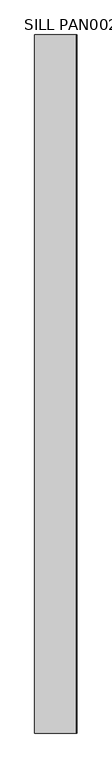
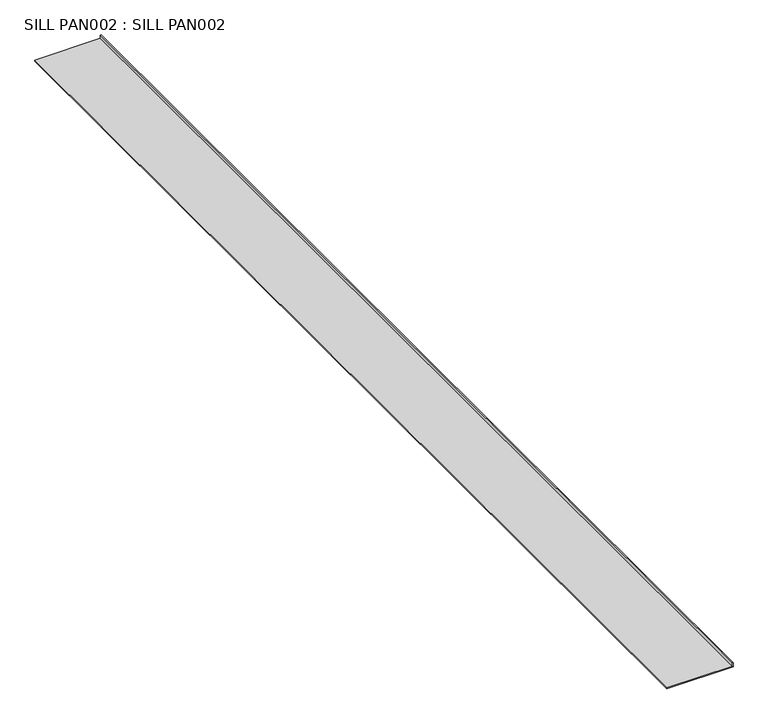
"""IFC4 building model written with IfcOpenShell, lengths in millimetres: proxy geometry, SILL PAN002 : SILL PAN002."""

from ifc_helpers import new_model, si_unit, frame, origin, place, context, project, spatial, polyline, outline, extrude, source, transform, mapped, element, save


def sill_pan002_sill_pan002_29912948(model_context):
    return source(origin(), model_context, "Body", "SweptSolid", [
        extrude(outline(polyline([(42765.4289739, 6057.1612048), (42763.8414739, 6057.1612048), (42763.8414739, 6178.6035156), (42771.7794904, 6178.6035156), (42771.7794904, 6177.0158698), (42765.4289739, 6177.0158698), (42765.4289739, 6057.1612048)])), frame((0.0, -1052.8908926, 0.0), z_axis=(0.0, 1.0, 0.0), x_axis=(0.0, 0.0, 1.0)), (0.0, 0.0, 1.0), 1999.85),
    ])


if __name__ == "__main__":
    model = new_model("IFC4")
    model_context = context("Model", 3, world=origin())
    ifc_project = project(units=[si_unit("LENGTHUNIT", "METRE", prefix="MILLI")], contexts=[model_context])
    site = spatial("IfcSite", under=ifc_project)
    building = spatial("IfcBuilding", under=site)
    placement = place(None, origin())
    sill_pan002_sill_pan002_shape = sill_pan002_sill_pan002_29912948(model_context)
    element("IfcBuildingElementProxy", 1, Name="SILL PAN002 : SILL PAN002", ObjectType="SILL PAN002 : SILL PAN002", at=placement, inside=building, context=model_context, shape_type="MappedRepresentation", body=[
        mapped(sill_pan002_sill_pan002_shape, transform((0.0, 0.0, 0.0), x_axis=(1.0, 0.0, 0.0), y_axis=(0.0, 1.0, 0.0), z_axis=(0.0, 0.0, 1.0))),
    ])
    save(model, "model.ifc")

# Revit data of these elements
# Type "SILL PAN002 : SILL PAN002"
#   NameOverride = "SILL PAN002"
# Element 1 (IfcBuildingElementProxy, "SILL PAN002 : SILL PAN002")
#   Materials on its faces: "COPPER SILL PAN AT ALL EXTERIOR WINDOWS/DOORS PER DETAIL 1/A4.1"
# Materials
#   "COPPER SILL PAN AT ALL EXTERIOR WINDOWS/DOORS PER DETAIL 1/A4.1": class "Unassigned", colour RGB 255 170 255, transparency 0, Cost = 0
